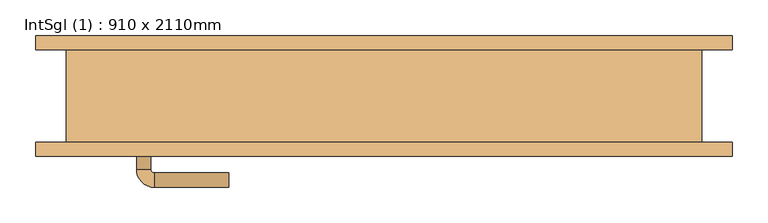
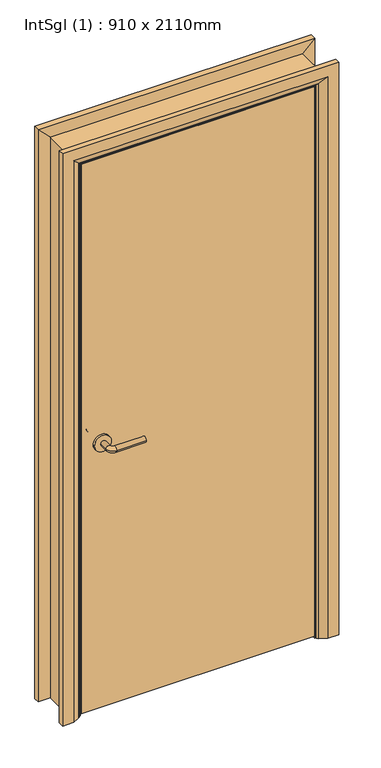
"""IFC4 building model written with IfcOpenShell, lengths in millimetres: door geometry, IntSgl (1) : 910 x 2110mm."""

from ifc_helpers import new_model, si_unit, point, frame, frame_2d, origin, place, context, project, spatial, polyline, circle_curve, ellipse_curve, trimmed, segment, composite_curve, outline, extrude, faceted_brep, source, transform, mapped, element, save
from ifc_brep_helpers import plane_surface, cylinder_surface, revolved_surface, advanced_brep


def intsgl_1_910_x_2110mm_ad2476ae(model_context):
    return source(origin(), model_context, "Body", "SolidModel", [
        advanced_brep(
        [(-348.0, -19.0, 1000.0), (-328.0, -19.0, 1000.0), (-348.0, 11.0, 1000.0), (-328.0, 11.0, 1000.0), (-323.0, 16.0, 1000.0), (-323.0, 36.0, 1000.0), (-218.0, 36.0, 1000.0), (-218.0, 16.0, 1000.0)],
        [
            (0, 1, circle_curve(frame((-338.0, -19.0, 1000.0), z_axis=(0.0, -1.0, 0.0), x_axis=(1.0, 0.0, 0.0)), 10.0)),
            (1, 0, circle_curve(frame((-338.0, -19.0, 1000.0), z_axis=(0.0, -1.0, 0.0), x_axis=(1.0, 0.0, 0.0)), 10.0)),
            (0, 2),
            (2, 3, circle_curve(frame((-338.0, 11.0, 1000.0), z_axis=(0.0, -1.0, 0.0), x_axis=(1.0, 0.0, 0.0)), 10.0)),
            (3, 1),
            (3, 2, circle_curve(frame((-338.0, 11.0, 1000.0), z_axis=(0.0, -1.0, 0.0), x_axis=(1.0, 0.0, 0.0)), 10.0)),
            (4, 3, circle_curve(frame((-323.0, 11.0, 1000.0), z_axis=(0.0, 0.0, 1.0), x_axis=(-1.0, 0.0, 0.0)), 5.0)),
            (2, 5, circle_curve(frame((-323.0, 11.0, 1000.0), z_axis=(0.0, 0.0, -1.0), x_axis=(-1.0, 0.0, 0.0)), 25.0)),
            (5, 4, circle_curve(frame((-323.0, 26.0, 1000.0), z_axis=(-1.0, 0.0, 0.0), x_axis=(0.0, -1.0, 0.0)), 10.0)),
            (4, 5, circle_curve(frame((-323.0, 26.0, 1000.0), z_axis=(-1.0, 0.0, 0.0), x_axis=(0.0, -1.0, 0.0)), 10.0)),
            (6, 7, circle_curve(frame((-218.0, 26.0, 1000.0), z_axis=(1.0, 0.0, 0.0), x_axis=(0.0, -1.0, 0.0)), 10.0)),
            (7, 6, circle_curve(frame((-218.0, 26.0, 1000.0), z_axis=(1.0, 0.0, 0.0), x_axis=(0.0, -1.0, 0.0)), 10.0)),
            (5, 6),
            (7, 4),
        ],
        [
            plane_surface(frame((-338.0, -19.0, 1000.0), z_axis=(0.0, -1.0, 0.0), x_axis=(0.0, 0.0, 1.0))),
            cylinder_surface(frame((-338.0, -19.0, 1000.0), z_axis=(0.0, -1.0, 0.0), x_axis=(1.0, 0.0, 0.0)), 10.0),
            revolved_surface(trimmed(ellipse_curve(frame((-338.0, 11.0, 1000.0), z_axis=(0.0, -1.0, 0.0), x_axis=(1.0, 0.0, 0.0)), 10.0, 10.0), [point((-348.0, 11.0, 1000.0))], [point((-328.0, 11.0, 1000.0))], True, "CARTESIAN"), (-323.0, 11.0, 1000.0), (0.0, 0.0, -1.0)),
            revolved_surface(trimmed(ellipse_curve(frame((-338.0, 11.0, 1000.0), z_axis=(0.0, -1.0, 0.0), x_axis=(1.0, 0.0, 0.0)), 10.0, 10.0), [point((-328.0, 11.0, 1000.0))], [point((-348.0, 11.0, 1000.0))], True, "CARTESIAN"), (-323.0, 11.0, 1000.0), (0.0, 0.0, -1.0)),
            plane_surface(frame((-218.0, 26.0, 1000.0), z_axis=(1.0, 0.0, 0.0), x_axis=(0.0, 0.0, 1.0))),
            cylinder_surface(frame((-323.0, 26.0, 1000.0), z_axis=(-1.0, 0.0, 0.0), x_axis=(0.0, -1.0, 0.0)), 10.0),
        ],
        [
            (0, [[1, 2]]),
            (1, [[-1, 3, 4, 5]]),
            (1, [[-2, -5, 6, -3]]),
            (2, [[7, -4, 8, 9]]),
            (3, [[-8, -6, -7, 10]]),
            (4, [[11, 12]]),
            (5, [[-9, 13, -12, 14]]),
            (5, [[-10, -14, -11, -13]]),
        ],
    ),
        extrude(outline(composite_curve([segment(trimmed(circle_curve(frame_2d((1000.0, -340.5)), 30.0), [point((1000.0, -370.5))], [point((1000.0, -310.5))], False, "CARTESIAN"), True, "CONTINUOUS"), segment(trimmed(circle_curve(frame_2d((1000.0, -340.5)), 30.0), [point((1000.0, -310.5))], [point((1000.0, -370.5))], False, "CARTESIAN"), True, "CONTINUOUS")], self_intersect=False)), frame((0.0, -27.0, 0.0), z_axis=(0.0, 1.0, 0.0), x_axis=(0.0, 0.0, 1.0)), (0.0, 0.0, 1.0), 8.0),
        advanced_brep(
        [(-348.0, -73.0, 1000.0), (-328.0, -73.0, 1000.0), (-328.0, -103.0, 1000.0), (-348.0, -103.0, 1000.0), (-323.0, -108.0, 1000.0), (-323.0, -128.0, 1000.0), (-218.0, -128.0, 1000.0), (-218.0, -108.0, 1000.0)],
        [
            (0, 1, circle_curve(frame((-338.0, -73.0, 1000.0), z_axis=(0.0, 1.0, 0.0), x_axis=(1.0, 0.0, 0.0)), 10.0)),
            (1, 0, circle_curve(frame((-338.0, -73.0, 1000.0), z_axis=(0.0, 1.0, 0.0), x_axis=(1.0, 0.0, 0.0)), 10.0)),
            (1, 2),
            (2, 3, circle_curve(frame((-338.0, -103.0, 1000.0), z_axis=(0.0, 1.0, 0.0), x_axis=(1.0, 0.0, 0.0)), 10.0)),
            (3, 0),
            (3, 2, circle_curve(frame((-338.0, -103.0, 1000.0), z_axis=(0.0, 1.0, 0.0), x_axis=(1.0, 0.0, 0.0)), 10.0)),
            (4, 5, circle_curve(frame((-323.0, -118.0, 1000.0), z_axis=(-1.0, 0.0, 0.0), x_axis=(0.0, 1.0, 0.0)), 10.0)),
            (5, 3, circle_curve(frame((-323.0, -103.0, 1000.0), z_axis=(0.0, 0.0, -1.0), x_axis=(-1.0, 0.0, 0.0)), 25.0)),
            (2, 4, circle_curve(frame((-323.0, -103.0, 1000.0), z_axis=(0.0, 0.0, 1.0), x_axis=(-1.0, 0.0, 0.0)), 5.0)),
            (5, 4, circle_curve(frame((-323.0, -118.0, 1000.0), z_axis=(-1.0, 0.0, 0.0), x_axis=(0.0, 1.0, 0.0)), 10.0)),
            (6, 7, circle_curve(frame((-218.0, -118.0, 1000.0), z_axis=(1.0, 0.0, 0.0), x_axis=(0.0, 1.0, 0.0)), 10.0)),
            (7, 6, circle_curve(frame((-218.0, -118.0, 1000.0), z_axis=(1.0, 0.0, 0.0), x_axis=(0.0, 1.0, 0.0)), 10.0)),
            (4, 7),
            (6, 5),
        ],
        [
            plane_surface(frame((-338.0, -73.0, 1000.0), z_axis=(0.0, 1.0, 0.0), x_axis=(0.0, 0.0, 1.0))),
            cylinder_surface(frame((-338.0, -73.0, 1000.0), z_axis=(0.0, 1.0, 0.0), x_axis=(1.0, 0.0, 0.0)), 10.0),
            revolved_surface(trimmed(ellipse_curve(frame((-338.0, -103.0, 1000.0), z_axis=(0.0, -1.0, 0.0), x_axis=(1.0, 0.0, 0.0)), 10.0, 10.0), [point((-348.0, -103.0, 1000.0))], [point((-328.0, -103.0, 1000.0))], True, "CARTESIAN"), (-323.0, -103.0, 1000.0), (0.0, 0.0, -1.0)),
            revolved_surface(trimmed(ellipse_curve(frame((-338.0, -103.0, 1000.0), z_axis=(0.0, -1.0, 0.0), x_axis=(1.0, 0.0, 0.0)), 10.0, 10.0), [point((-328.0, -103.0, 1000.0))], [point((-348.0, -103.0, 1000.0))], True, "CARTESIAN"), (-323.0, -103.0, 1000.0), (0.0, 0.0, -1.0)),
            plane_surface(frame((-218.0, -118.0, 1000.0), z_axis=(1.0, 0.0, 0.0), x_axis=(0.0, 0.0, 1.0))),
            cylinder_surface(frame((-323.0, -118.0, 1000.0), z_axis=(-1.0, 0.0, 0.0), x_axis=(0.0, 1.0, 0.0)), 10.0),
        ],
        [
            (0, [[1, 2]]),
            (1, [[3, 4, 5, -2]]),
            (1, [[-5, 6, -3, -1]]),
            (2, [[7, 8, -4, 9]]),
            (3, [[10, -9, -6, -8]]),
            (4, [[11, 12]]),
            (5, [[13, -11, 14, -7]]),
            (5, [[-14, -12, -13, -10]]),
        ],
    ),
        extrude(outline(composite_curve([segment(trimmed(circle_curve(frame_2d((1000.0, -340.5)), 30.0), [point((1000.0, -370.5))], [point((1000.0, -310.5))], False, "CARTESIAN"), True, "CONTINUOUS"), segment(trimmed(circle_curve(frame_2d((1000.0, -340.5)), 30.0), [point((1000.0, -310.5))], [point((1000.0, -370.5))], False, "CARTESIAN"), True, "CONTINUOUS")], self_intersect=False)), frame((0.0, -73.0, 0.0), z_axis=(0.0, 1.0, 0.0), x_axis=(0.0, 0.0, 1.0)), (0.0, 0.0, 1.0), 8.0),
        extrude(outline(polyline([(413.0, -27.0), (413.0, -65.0), (-413.0, -65.0), (-413.0, -27.0), (413.0, -27.0)])), frame((0.0, 0.0, 8.0), z_axis=(0.0, 0.0, 1.0), x_axis=(1.0, 0.0, 0.0)), (0.0, 0.0, 1.0), 2060.0),
        advanced_brep(
        [(490.0, -85.0, 0.0), (450.0, -85.0, 0.0), (424.0, -71.0, 0.0), (420.0, -65.0, 0.0), (490.0, -65.0, 0.0), (490.0, -65.0, 2145.0), (490.0, -85.0, 2145.0), (420.0, -65.0, 2075.0), (-420.0, -65.0, 2075.0), (-420.0, -65.0, 0.0), (-490.0, -65.0, 0.0), (-490.0, -65.0, 2145.0), (424.0, -71.0, 2079.0), (450.0, -85.0, 2105.0), (-490.0, -85.0, 2145.0), (-490.0, -85.0, 0.0), (-450.0, -85.0, 0.0), (-450.0, -85.0, 2105.0), (-424.0, -71.0, 2079.0), (-424.0, -71.0, 0.0)],
        [
            (0, 1),
            (1, 2),
            (2, 3, circle_curve(frame((428.0, -64.0, 0.0), z_axis=(0.0, 0.0, -1.0), x_axis=(1.0, 0.0, 0.0)), 8.0622577)),
            (3, 4),
            (4, 0),
            (4, 5),
            (5, 6),
            (6, 0),
            (3, 7),
            (7, 8),
            (8, 9),
            (9, 10),
            (10, 11),
            (11, 5),
            (2, 12),
            (12, 7, ellipse_curve(frame((428.0, -64.0, 2083.0), z_axis=(0.7071067811865475, 0.0, -0.7071067811865475), x_axis=(-0.7071067811865474, 0.0, -0.7071067811865476)), 11.4017543, 8.0622577)),
            (1, 13),
            (13, 12),
            (6, 14),
            (14, 15),
            (15, 16),
            (16, 17),
            (17, 13),
            (11, 14),
            (12, 18),
            (18, 8, ellipse_curve(frame((-428.0, -64.0, 2083.0), z_axis=(0.7071067811865475, 0.0, 0.7071067811865475), x_axis=(0.7071067811865476, 0.0, -0.7071067811865474)), 11.4017543, 8.0622577)),
            (17, 18),
            (15, 10),
            (9, 19, circle_curve(frame((-428.0, -64.0, 0.0), z_axis=(0.0, 0.0, -1.0), x_axis=(-1.0, 0.0, 0.0)), 8.0622577)),
            (19, 16),
            (18, 19),
        ],
        [
            plane_surface(frame((420.0, -65.0, 0.0), z_axis=(0.0, 0.0, -1.0), x_axis=(0.0, 1.0, 0.0))),
            plane_surface(frame((490.0, -85.0, 0.0), z_axis=(1.0, 0.0, 0.0), x_axis=(0.0, 0.0, 1.0))),
            plane_surface(frame((490.0, -65.0, 0.0), z_axis=(0.0, 1.0, 0.0), x_axis=(0.0, 0.0, 1.0))),
            cylinder_surface(frame((428.0, -64.0, 0.0), z_axis=(0.0, 0.0, -1.0), x_axis=(1.0, 0.0, 0.0)), 8.0622577),
            plane_surface(frame((424.0, -71.0, 0.0), z_axis=(-0.4740998230350126, -0.880471099922178, 0.0), x_axis=(0.0, 0.0, 1.0))),
            plane_surface(frame((450.0, -85.0, 0.0), z_axis=(0.0, -1.0, 0.0), x_axis=(0.0, 0.0, 1.0))),
            plane_surface(frame((490.0, -85.0, 2145.0), z_axis=(0.0, 0.0, 1.0), x_axis=(-1.0, 0.0, 0.0))),
            cylinder_surface(frame((420.0, -64.0, 2083.0), z_axis=(1.0, 0.0, 0.0), x_axis=(0.0, 0.0, 1.0)), 8.0622577),
            plane_surface(frame((424.0, -71.0, 2079.0), z_axis=(0.0, -0.8804710999221764, -0.4740998230350154), x_axis=(-1.0, 0.0, 0.0))),
            plane_surface(frame((-420.0, -65.0, 0.0), z_axis=(0.0, 0.0, -1.0), x_axis=(0.0, 1.0, 0.0))),
            plane_surface(frame((-490.0, -85.0, 2145.0), z_axis=(-1.0, 0.0, 0.0), x_axis=(0.0, 0.0, -1.0))),
            cylinder_surface(frame((-428.0, -64.0, 2075.0), z_axis=(0.0, 0.0, 1.0), x_axis=(-1.0, 0.0, 0.0)), 8.0622577),
            plane_surface(frame((-424.0, -71.0, 2079.0), z_axis=(0.47409982303501824, -0.8804710999221749, 0.0), x_axis=(0.0, 0.0, -1.0))),
        ],
        [
            (0, [[1, 2, 3, 4, 5]]),
            (1, [[6, 7, 8, -5]]),
            (2, [[9, 10, 11, 12, 13, 14, -6, -4]]),
            (3, [[15, 16, -9, -3]]),
            (4, [[17, 18, -15, -2]]),
            (5, [[-8, 19, 20, 21, 22, 23, -17, -1]]),
            (6, [[-14, 24, -19, -7]]),
            (7, [[25, 26, -10, -16]]),
            (8, [[-23, 27, -25, -18]]),
            (9, [[28, -12, 29, 30, -21]]),
            (10, [[-13, -28, -20, -24]]),
            (11, [[31, -29, -11, -26]]),
            (12, [[-22, -30, -31, -27]]),
        ],
    ),
        extrude(outline(polyline([(0.0, -396.0), (2051.0, -396.0), (2051.0, 396.0), (0.0, 396.0), (0.0, 415.0), (2070.0, 415.0), (2070.0, -415.0), (0.0, -415.0), (0.0, -396.0)])), frame((0.0, -25.0, 0.0), z_axis=(0.0, 1.0, 0.0), x_axis=(0.0, 0.0, 1.0)), (0.0, 0.0, 1.0), 32.0),
        advanced_brep(
        [(-490.0, 85.0, 0.0), (-450.0, 85.0, 0.0), (-424.0, 71.0, 0.0), (-420.0, 65.0, 0.0), (-490.0, 65.0, 0.0), (-490.0, 65.0, 2145.0), (-490.0, 85.0, 2145.0), (-420.0, 65.0, 2075.0), (-424.0, 71.0, 2079.0), (-450.0, 85.0, 2105.0), (490.0, 65.0, 2145.0), (490.0, 85.0, 2145.0), (420.0, 65.0, 2075.0), (424.0, 71.0, 2079.0), (450.0, 85.0, 2105.0), (490.0, 85.0, 0.0), (490.0, 65.0, 0.0), (420.0, 65.0, 0.0), (424.0, 71.0, 0.0), (450.0, 85.0, 0.0)],
        [
            (0, 1),
            (1, 2),
            (2, 3, circle_curve(frame((-428.0, 64.0, 0.0), z_axis=(0.0, 0.0, -1.0), x_axis=(-1.0, 0.0, 0.0)), 8.0622577)),
            (3, 4),
            (4, 0),
            (4, 5),
            (5, 6),
            (6, 0),
            (3, 7),
            (7, 5),
            (2, 8),
            (8, 7, ellipse_curve(frame((-428.0, 64.0, 2083.0), z_axis=(-0.7071067811865475, 0.0, -0.7071067811865475), x_axis=(0.7071067811865474, 0.0, -0.7071067811865476)), 11.4017543, 8.0622577)),
            (1, 9),
            (9, 8),
            (6, 9),
            (5, 10),
            (10, 11),
            (11, 6),
            (7, 12),
            (12, 10),
            (8, 13),
            (13, 12, ellipse_curve(frame((428.0, 64.0, 2083.0), z_axis=(-0.7071067811865475, 0.0, 0.7071067811865475), x_axis=(-0.7071067811865476, 0.0, -0.7071067811865474)), 11.4017543, 8.0622577)),
            (9, 14),
            (14, 13),
            (11, 14),
            (15, 16),
            (16, 17),
            (17, 18, circle_curve(frame((428.0, 64.0, 0.0), z_axis=(0.0, 0.0, -1.0), x_axis=(1.0, 0.0, 0.0)), 8.0622577)),
            (18, 19),
            (19, 15),
            (10, 16),
            (15, 11),
            (12, 17),
            (13, 18),
            (14, 19),
        ],
        [
            plane_surface(frame((-420.0, 137.8010989, 0.0), z_axis=(0.0, 0.0, -1.0), x_axis=(1.0, 0.0, 0.0))),
            plane_surface(frame((-490.0, 85.0, 0.0), z_axis=(-1.0, 0.0, 0.0), x_axis=(0.0, 0.0, 1.0))),
            plane_surface(frame((-490.0, 65.0, 0.0), z_axis=(0.0, -1.0, 0.0), x_axis=(0.0, 0.0, 1.0))),
            cylinder_surface(frame((-428.0, 64.0, 0.0), z_axis=(0.0, 0.0, -1.0), x_axis=(-1.0, 0.0, 0.0)), 8.0622577),
            plane_surface(frame((-424.0, 71.0, 0.0), z_axis=(0.4740998230350183, 0.8804710999221749, 0.0), x_axis=(0.0, 0.0, 1.0))),
            plane_surface(frame((-450.0, 85.0, 0.0), z_axis=(0.0, 1.0, 0.0), x_axis=(0.0, 0.0, 1.0))),
            plane_surface(frame((-490.0, 85.0, 2145.0), z_axis=(0.0, 0.0, 1.0), x_axis=(1.0, 0.0, 0.0))),
            plane_surface(frame((-490.0, 65.0, 2145.0), z_axis=(0.0, -1.0, 0.0), x_axis=(1.0, 0.0, 0.0))),
            cylinder_surface(frame((-420.0, 64.0, 2083.0), z_axis=(-1.0, 0.0, 0.0), x_axis=(0.0, 0.0, 1.0)), 8.0622577),
            plane_surface(frame((-424.0, 71.0, 2079.0), z_axis=(0.0, 0.8804710999221749, -0.4740998230350183), x_axis=(1.0, 0.0, 0.0))),
            plane_surface(frame((-450.0, 85.0, 2105.0), z_axis=(0.0, 1.0, 0.0), x_axis=(1.0, 0.0, 0.0))),
            plane_surface(frame((420.0, 137.8010989, 0.0), z_axis=(0.0, 0.0, -1.0), x_axis=(-1.0, 0.0, 0.0))),
            plane_surface(frame((490.0, 85.0, 2145.0), z_axis=(1.0, 0.0, 0.0), x_axis=(0.0, 0.0, -1.0))),
            plane_surface(frame((490.0, 65.0, 2145.0), z_axis=(0.0, -1.0, 0.0), x_axis=(0.0, 0.0, -1.0))),
            cylinder_surface(frame((428.0, 64.0, 2075.0), z_axis=(0.0, 0.0, 1.0), x_axis=(1.0, 0.0, 0.0)), 8.0622577),
            plane_surface(frame((424.0, 71.0, 2079.0), z_axis=(-0.4740998230350183, 0.8804710999221749, 0.0), x_axis=(0.0, 0.0, -1.0))),
            plane_surface(frame((450.0, 85.0, 2105.0), z_axis=(0.0, 1.0, 0.0), x_axis=(0.0, 0.0, -1.0))),
        ],
        [
            (0, [[1, 2, 3, 4, 5]]),
            (1, [[6, 7, 8, -5]]),
            (2, [[9, 10, -6, -4]]),
            (3, [[11, 12, -9, -3]]),
            (4, [[13, 14, -11, -2]]),
            (5, [[-8, 15, -13, -1]]),
            (6, [[16, 17, 18, -7]]),
            (7, [[19, 20, -16, -10]]),
            (8, [[21, 22, -19, -12]]),
            (9, [[23, 24, -21, -14]]),
            (10, [[-18, 25, -23, -15]]),
            (11, [[26, 27, 28, 29, 30]]),
            (12, [[31, -26, 32, -17]]),
            (13, [[33, -27, -31, -20]]),
            (14, [[34, -28, -33, -22]]),
            (15, [[35, -29, -34, -24]]),
            (16, [[-32, -30, -35, -25]]),
        ],
    ),
        faceted_brep([(-415.0, -65.0, 0.0), (-447.0, -65.0, 0.0), (-447.0, 65.0, 0.0), (-415.0, 65.0, 0.0), (-415.0, 65.0, 2070.0), (-415.0, -65.0, 2070.0), (-447.0, 65.0, 2102.0), (-447.0, -65.0, 2102.0), (415.0, 65.0, 2070.0), (415.0, -65.0, 2070.0), (447.0, 65.0, 2102.0), (447.0, -65.0, 2102.0), (415.0, -65.0, 0.0), (415.0, 65.0, 0.0), (447.0, 65.0, 0.0), (447.0, -65.0, 0.0)], [[[0, 1, 2, 3]], [[3, 4, 5, 0]], [[2, 6, 4, 3]], [[1, 7, 6, 2]], [[0, 5, 7, 1]], [[4, 8, 9, 5]], [[6, 10, 8, 4]], [[7, 11, 10, 6]], [[5, 9, 11, 7]], [[12, 13, 14, 15]], [[8, 13, 12, 9]], [[10, 14, 13, 8]], [[11, 15, 14, 10]], [[9, 12, 15, 11]]]),
    ])


if __name__ == "__main__":
    model = new_model("IFC4")
    model_context = context("Model", 3, world=origin())
    ifc_project = project(units=[si_unit("LENGTHUNIT", "METRE", prefix="MILLI")], contexts=[model_context])
    site = spatial("IfcSite", under=ifc_project)
    building = spatial("IfcBuilding", under=site)
    placement = place(None, origin())
    intsgl_1_910_x_2110mm_shape = intsgl_1_910_x_2110mm_ad2476ae(model_context)
    element("IfcDoor", 1, ObjectType="IntSgl (1) : 910 x 2110mm", at=placement, inside=building, context=model_context, shape_type="MappedRepresentation", body=[
        mapped(intsgl_1_910_x_2110mm_shape, transform((0.0, 0.0, 0.0), x_axis=(1.0, 0.0, 0.0), y_axis=(0.0, 1.0, 0.0), z_axis=(0.0, 0.0, 1.0))),
    ])
    save(model, "model.ifc")

# Revit data of these elements
# Type "IntSgl (1) : 910 x 2110mm"
#   Construction Type Id = "MDOOR"
#   Analytic Construction = "Metal"
#   Type Mark = "41"
#   Type Comments = "Internal Single"
#   Operation = "SingleSwingRight"
#   Manufacturer = "Revit"
#   Keynote = "L20"
#   Description = "Internal Single Door"
#   Visual Light Transmittance = 0
#   Solar Heat Gain Coefficient = 0
#   Heat Transfer Coefficient (U) = 3.7021 W/(m²·K)
#   UnderCut = 8 mm
#   Tolerance = 2 mm
#   Thickness = 38 mm
#   Structural Tolerance = 8 mm
#   StopDepth = 32 mm
#   Stop Thickness = 19 mm
#   Rough Width = 910 mm
#   Rough Height = 2110 mm
#   Height to Top Lock Rail = 1000 mm
#   Handle Z Distance = 1000 mm
#   Handle X Distance = 75 mm
#   Frame Thickness = 32 mm
#   Door Panel Width = 826 mm
#   Door Panel Thickness = 38 mm
#   Door Panel Offset = 0 mm
#   Height = 2110 mm
#   Width = 910 mm
#   Door Panel Height = 2060 mm
#   Architrave Setback = 5 mm
#   Function = 0
#   Vis - Ironmongery = yes
#   Material Ironmongery = Door - Handle
#   Material Frame = Door - Frame/Mullion (1)
#   Material Door = Door - Panel
#   Material Architrave = Door - Architrave
#   Wall Closure = (empty or 0)
# Element 1 (IfcDoor, "IntSgl (1) : 910 x 2110mm")
#   Materials on its faces: "Door - Architrave", "Door - Handle", "Door - Frame/Mullion (1)", "Door - Panel"
# Materials
#   "Door - Handle": class "Miscellaneous", colour RGB 0 0 0, transparency 0, Keynote = "P21"
#   "Door - Frame/Mullion (1)": class "Wood", colour RGB 212 179 113, transparency 0, Keynote = "L20", Cost = 0
#   "Door - Panel": class "Wood", colour RGB 210 159 95, transparency 0, Keynote = "L20"
#   "Door - Architrave": class "Wood", colour RGB 154 90 5, transparency 0, Keynote = "P20"
